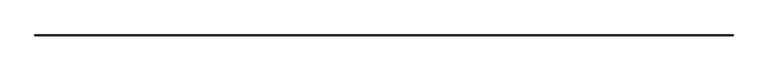
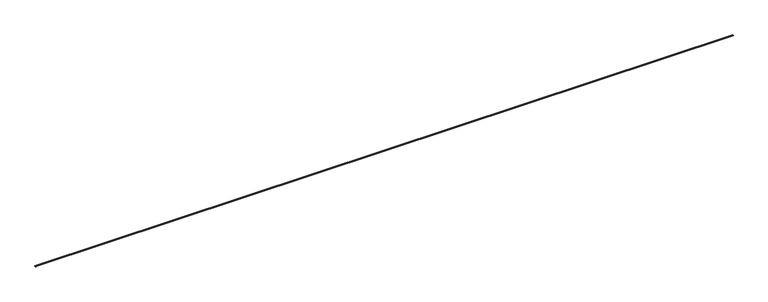
"""IFC4 building model written with IfcOpenShell, lengths in millimetres: proxy geometry, Generic Models 3:Generic Models 1:4:Generic Models 1:4 : Generic Models 3:Generic Models 1:300625:1:Generic Models 1:4:Generic Models 1:4 : Generic Models 3:Generic Models 1:300625:1 : Generic Models 3:Generic Models 1:4:Generic Models 1:4 : Generic Models 3:Generic Models 1:300625:338780:3 : Generic Models 3:Generic Models 1:4:Generic Models 1:4 : Generic Models 3:Generic Models 1:300625:1:Generic Models 1:4:Generic Models 1:4 : Generic Models 3:Generic Models 1:300625:1 : Generic Models 3:Generic Models 1:4:Generic Models 1:4 : Generic Models 3:Generic Models 1:300625:338780:317135."""

from ifc_helpers import new_model, si_unit, frame, origin, place, context, project, spatial, polyline, outline, extrude, source, transform, mapped, element, save


def generic_models_bd1f5dd9(model_context):
    return source(origin(), model_context, "Body", "SweptSolid", [
        extrude(outline(polyline([(-579088.4739295, 3712.8072545), (-579094.6612723, 3712.8072545), (-579094.1146795, 3713.4586585), (-579093.8638533, 3714.3947545), (-579094.1146795, 3715.3308505), (-579094.6612723, 3715.9822545), (-579088.4739295, 3715.9822545), (-579089.0205223, 3715.3308505), (-579089.2713485, 3714.3947545), (-579089.0205223, 3713.4586585), (-579088.4739295, 3712.8072545)])), frame((591306.0367239, 0.0, 0.0), z_axis=(1.0, 0.0, 0.0), x_axis=(0.0, 1.0, 0.0)), (0.0, 0.0, 1.0), 4876.8),
    ])


if __name__ == "__main__":
    model = new_model("IFC4")
    model_context = context("Model", 3, world=origin())
    ifc_project = project(units=[si_unit("LENGTHUNIT", "METRE", prefix="MILLI")], contexts=[model_context])
    site = spatial("IfcSite", under=ifc_project)
    building = spatial("IfcBuilding", under=site)
    placement = place(None, origin())
    generic_models_shape = generic_models_bd1f5dd9(model_context)
    element("IfcBuildingElementProxy", 1, Name="Generic Models 3:Generic Models 1:4:Generic Models 1:4 : Generic Models 3:Generic Models 1:300625:1:Generic Models 1:4:Generic Models 1:4 : Generic Models 3:Generic Models 1:300625:1 : Generic Models 3:Generic Models 1:4:Generic Models 1:4 : Generic Models 3:Generic Models 1:300625:338780:3 : Generic Models 3:Generic Models 1:4:Generic Models 1:4 : Generic Models 3:Generic Models 1:300625:1:Generic Models 1:4:Generic Models 1:4 : Generic Models 3:Generic Models 1:300625:1 : Generic Models 3:Generic Models 1:4:Generic Models 1:4 : Generic Models 3:Generic Models 1:300625:338780:317135", ObjectType="Generic Models 3:Generic Models 1:4:Generic Models 1:4 : Generic Models 3:Generic Models 1:300625:1:Generic Models 1:4:Generic Models 1:4 : Generic Models 3:Generic Models 1:300625:1 : Generic Models 3:Generic Models 1:4:Generic Models 1:4 : Generic Models 3:Generic Models 1:300625:338780:3 : Generic Models 3:Generic Models 1:4:Generic Models 1:4 : Generic Models 3:Generic Models 1:300625:1:Generic Models 1:4:Generic Models 1:4 : Generic Models 3:Generic Models 1:300625:1 : Generic Models 3:Generic Models 1:4:Generic Models 1:4 : Generic Models 3:Generic Models 1:300625:338780:317135", at=placement, inside=building, context=model_context, shape_type="MappedRepresentation", body=[
        mapped(generic_models_shape, transform((0.0, 0.0, 0.0), x_axis=(1.0, 0.0, 0.0), y_axis=(0.0, 1.0, 0.0), z_axis=(0.0, 0.0, 1.0))),
    ])
    save(model, "model.ifc")

# Revit data of these elements
# Type "Generic Models 3:Generic Models 1:4:Generic Models 1:4 : Generic Models 3:Generic Models 1:300625:1:Generic Models 1:4:Generic Models 1:4 : Generic Models 3:Generic Models 1:300625:1 : Generic Models 3:Generic Models 1:4:Generic Models 1:4 : Generic Models 3:Generic Models 1:300625:338780:3 : Generic Models 3:Generic Models 1:4:Generic Models 1:4 : Generic Models 3:Generic Models 1:300625:1:Generic Models 1:4:Generic Models 1:4 : Generic Models 3:Generic Models 1:300625:1 : Generic Models 3:Generic Models 1:4:Generic Models 1:4 : Generic Models 3:Generic Models 1:300625:338780:317135"
#   NameOverride = "Generic Models 3:Generic Models 1:4:Generic Models 1:4 : Generic Models 3:Generic Models 1:300625:1:Generic Models 1:4:Generic Models 1:4 : Generic Models 3:Generic Models 1:300625:1 : Generic Models 3:Generic Models 1:4:Generic Models 1:4 : Generic Models 3:Generic Models 1:300625:338780:317135"
#   ObjectTypeOverride = "Generic Models 1:4:Generic Models 1:4 : Generic Models 3:Generic Models 1:300625:1 : Generic Models 3:Generic Models 1:4:Generic Models 1:4 : Generic Models 3:Generic Models 1:300625:338780"
#   Reference = "Generic Models 1"
#   Tag = "317135"
# Element 1 (IfcBuildingElementProxy, "Generic Models 3:Generic Models 1:4:Generic Models 1:4 : Generic Models 3:Generic Models 1:300625:1:Generic Models 1:4:Generic Models 1:4 : Generic Models 3:Generic Models 1:300625:1 : Generic Models 3:Generic Models 1:4:Generic Models 1:4 : Generic Models 3:Generic Models 1:300625:338780:3 : Generic Models 3:Generic Models 1:4:Generic Models 1:4 : Generic Models 3:Generic Models 1:300625:1:Generic Models 1:4:Generic Models 1:4 : Generic Models 3:Generic Models 1:300625:1 : Generic Models 3:Generic Models 1:4:Generic Models 1:4 : Generic Models 3:Generic Models 1:300625:338780:317135")
#   Materials on its faces: "SEALANT & BACKER ROD"
# Materials
#   "SEALANT & BACKER ROD": class "Unassigned", colour RGB 120 120 120, transparency 0, Cost = 0
